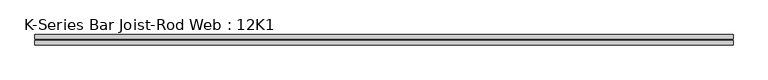
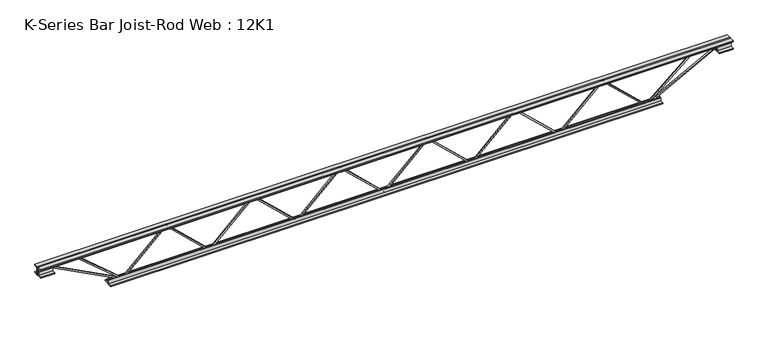
"""IFC4 building model written with IfcOpenShell, lengths in millimetres: beam geometry, K-Series Bar Joist-Rod Web : 12K1."""

from ifc_helpers import new_model, si_unit, frame, origin, place, context, project, spatial, polyline, outline, extrude, source, transform, mapped, element, save


def k_series_bar_joist_rod_web_12k1_562b93e1(model_context):
    return source(origin(), model_context, "Body", "SweptSolid", [
        extrude(outline(polyline([(-141.2875, 631.2958333), (-150.8125, 631.2958333), (-150.8125, 636.3642323), (141.2875, 945.662149), (141.2875, 948.225351), (-150.8125, 1257.5232677), (-150.8125, 1262.5916667), (-141.2875, 1262.5916667), (-141.2875, 1261.3100656), (150.8125, 952.012149), (150.8125, 941.875351), (-141.2875, 632.5774344), (-141.2875, 631.2958333)])), frame((0.0, -4.7625, 0.0), z_axis=(0.0, 1.0, 0.0), x_axis=(0.0, 0.0, 1.0)), (0.0, 0.0, 1.0), 9.525),
        extrude(outline(polyline([(-141.2875, 0.0), (-150.8125, 0.0), (-150.8125, 5.068399), (141.2875, 314.3663156), (141.2875, 316.9295177), (-150.8125, 626.2274344), (-150.8125, 631.2958333), (-141.2875, 631.2958333), (-141.2875, 630.0142323), (150.8125, 320.7163156), (150.8125, 310.5795177), (-141.2875, 1.281601), (-141.2875, 0.0)])), frame((0.0, -4.7625, 0.0), z_axis=(0.0, 1.0, 0.0), x_axis=(0.0, 0.0, 1.0)), (0.0, 0.0, 1.0), 9.525),
        extrude(outline(polyline([(-141.2875, -631.2958333), (-150.8125, -631.2958333), (-150.8125, -626.2274344), (141.2875, -316.9295177), (141.2875, -314.3663156), (-150.8125, -5.068399), (-150.8125, 0.0), (-141.2875, 0.0), (-141.2875, -1.281601), (150.8125, -310.5795177), (150.8125, -320.7163156), (-141.2875, -630.0142323), (-141.2875, -631.2958333)])), frame((0.0, -4.7625, 0.0), z_axis=(0.0, 1.0, 0.0), x_axis=(0.0, 0.0, 1.0)), (0.0, 0.0, 1.0), 9.525),
        extrude(outline(polyline([(-141.2875, -1262.5916667), (-150.8125, -1262.5916667), (-150.8125, -1257.5232677), (141.2875, -948.225351), (141.2875, -945.662149), (-150.8125, -636.3642323), (-150.8125, -631.2958333), (-141.2875, -631.2958333), (-141.2875, -632.5774344), (150.8125, -941.875351), (150.8125, -952.012149), (-141.2875, -1261.3100656), (-141.2875, -1262.5916667)])), frame((0.0, -4.7625, 0.0), z_axis=(0.0, 1.0, 0.0), x_axis=(0.0, 0.0, 1.0)), (0.0, 0.0, 1.0), 9.525),
        extrude(outline(polyline([(-141.2875, 1262.5916667), (-150.8125, 1262.5916667), (-150.8125, 1267.6600656), (141.2875, 1576.9579823), (141.2875, 1579.5211844), (-150.8125, 1888.819101), (-150.8125, 1893.8875), (-141.2875, 1893.8875), (-141.2875, 1892.605899), (150.8125, 1583.3079823), (150.8125, 1573.1711844), (-141.2875, 1263.8732677), (-141.2875, 1262.5916667)])), frame((0.0, -4.7625, 0.0), z_axis=(0.0, 1.0, 0.0), x_axis=(0.0, 0.0, 1.0)), (0.0, 0.0, 1.0), 9.525),
        extrude(outline(polyline([(-141.2875, -1893.8875), (-150.8125, -1893.8875), (-150.8125, -1888.819101), (141.2875, -1579.5211844), (141.2875, -1576.9579823), (-150.8125, -1267.6600656), (-150.8125, -1262.5916667), (-141.2875, -1262.5916667), (-141.2875, -1263.8732677), (150.8125, -1573.1711844), (150.8125, -1583.3079823), (-141.2875, -1892.605899), (-141.2875, -1893.8875)])), frame((0.0, -4.7625, 0.0), z_axis=(0.0, 1.0, 0.0), x_axis=(0.0, 0.0, 1.0)), (0.0, 0.0, 1.0), 9.525),
        extrude(outline(polyline([(4.7625, 152.4), (36.5125, 152.4), (36.5125, 146.05), (11.1125, 146.05), (11.1125, 120.65), (4.7625, 120.65), (4.7625, 152.4)])), frame((-2503.4875, 0.0, 0.0), z_axis=(1.0, 0.0, 0.0), x_axis=(0.0, 1.0, 0.0)), (0.0, 0.0, 1.0), 5006.975),
        extrude(outline(polyline([(-4.7625, 152.4), (-4.7625, 120.65), (-11.1125, 120.65), (-11.1125, 146.05), (-36.5125, 146.05), (-36.5125, 152.4), (-4.7625, 152.4)])), frame((-2503.4875, 0.0, 0.0), z_axis=(1.0, 0.0, 0.0), x_axis=(0.0, 1.0, 0.0)), (0.0, 0.0, 1.0), 5006.975),
        extrude(outline(polyline([(-4.7625, 88.9), (-36.5125, 88.9), (-36.5125, 95.25), (-11.1125, 95.25), (-11.1125, 120.65), (-4.7625, 120.65), (-4.7625, 88.9)])), frame((-2503.4875, 0.0, 0.0), z_axis=(1.0, 0.0, 0.0), x_axis=(0.0, 1.0, 0.0)), (0.0, 0.0, 1.0), 101.6),
        extrude(outline(polyline([(36.5125, 88.9), (4.7625, 88.9), (4.7625, 120.65), (11.1125, 120.65), (11.1125, 95.25), (36.5125, 95.25), (36.5125, 88.9)])), frame((-2503.4875, 0.0, 0.0), z_axis=(1.0, 0.0, 0.0), x_axis=(0.0, 1.0, 0.0)), (0.0, 0.0, 1.0), 101.6),
        extrude(outline(polyline([(4.7625, 88.9), (4.7625, 120.65), (11.1125, 120.65), (11.1125, 95.25), (36.5125, 95.25), (36.5125, 88.9), (4.7625, 88.9)])), frame((2401.8875, 0.0, 0.0), z_axis=(1.0, 0.0, 0.0), x_axis=(0.0, 1.0, 0.0)), (0.0, 0.0, 1.0), 101.6),
        extrude(outline(polyline([(-4.7625, 88.9), (-36.5125, 88.9), (-36.5125, 95.25), (-11.1125, 95.25), (-11.1125, 120.65), (-4.7625, 120.65), (-4.7625, 88.9)])), frame((2401.8875, 0.0, 0.0), z_axis=(1.0, 0.0, 0.0), x_axis=(0.0, 1.0, 0.0)), (0.0, 0.0, 1.0), 101.6),
        extrude(outline(polyline([(4.7625, -152.4), (4.7625, -120.65), (11.1125, -120.65), (11.1125, -146.05), (36.5125, -146.05), (36.5125, -152.4), (4.7625, -152.4)])), frame((-1995.4875, 0.0, 0.0), z_axis=(1.0, 0.0, 0.0), x_axis=(0.0, 1.0, 0.0)), (0.0, 0.0, 1.0), 3990.975),
        extrude(outline(polyline([(-4.7625, -152.4), (-36.5125, -152.4), (-36.5125, -146.05), (-11.1125, -146.05), (-11.1125, -120.65), (-4.7625, -120.65), (-4.7625, -152.4)])), frame((-1995.4875, 0.0, 0.0), z_axis=(1.0, 0.0, 0.0), x_axis=(0.0, 1.0, 0.0)), (0.0, 0.0, 1.0), 3990.975),
        extrude(outline(polyline([(0.0, -9.525), (0.0, 0.0), (573.7533355, 0.0), (573.7533355, -9.525), (0.0, -9.525)])), frame((-2404.1012714, 4.7625, 116.4332925), z_axis=(0.4648338989895134, 0.0, 0.8853979028381572), x_axis=(0.8853979028381572, 0.0, -0.4648338989895134)), (0.0, 0.0, 1.0), 9.525),
        extrude(outline(polyline([(0.0, -9.525), (0.0, 0.0), (413.2341918, 0.0), (413.2341918, -9.525), (0.0, -9.525)])), frame((-2212.6091186, 4.7625, 117.0121761), z_axis=(0.6453967393642932, 0.0, 0.7638475298238114), x_axis=(0.7638475298238114, 0.0, -0.6453967393642932)), (0.0, 0.0, 1.0), 9.525),
        extrude(outline(polyline([(0.0, -9.525), (0.0, 0.0), (573.7533355, 0.0), (573.7533355, -9.525), (0.0, -9.525)])), frame((2404.1012714, -4.7625, 116.4332925), z_axis=(-0.46483389898949556, 0.0, 0.8853979028381666), x_axis=(-0.8853979028381666, 0.0, -0.46483389898949556)), (0.0, 0.0, 1.0), 9.525),
        extrude(outline(polyline([(0.0, -9.525), (0.0, 0.0), (413.2341918, 0.0), (413.2341918, -9.525), (0.0, -9.525)])), frame((2212.6091186, -4.7625, 117.0121761), z_axis=(-0.6453967393642873, 0.0, 0.7638475298238165), x_axis=(-0.7638475298238165, 0.0, -0.6453967393642873)), (0.0, 0.0, 1.0), 9.525),
    ])


if __name__ == "__main__":
    model = new_model("IFC4")
    model_context = context("Model", 3, world=origin())
    ifc_project = project(units=[si_unit("LENGTHUNIT", "METRE", prefix="MILLI")], contexts=[model_context])
    site = spatial("IfcSite", under=ifc_project)
    building = spatial("IfcBuilding", under=site)
    placement = place(None, origin())
    k_series_bar_joist_rod_web_12k1_shape = k_series_bar_joist_rod_web_12k1_562b93e1(model_context)
    element("IfcBeam", 1, ObjectType="K-Series Bar Joist-Rod Web : 12K1", at=placement, inside=building, context=model_context, shape_type="MappedRepresentation", body=[
        mapped(k_series_bar_joist_rod_web_12k1_shape, transform((0.0, 0.0, 0.0), x_axis=(1.0, 0.0, 0.0), y_axis=(0.0, 1.0, 0.0), z_axis=(0.0, 0.0, 1.0))),
    ])
    save(model, "model.ifc")

# Revit data of these elements
# Type "K-Series Bar Joist-Rod Web : 12K1"
#   Assembly Code = "B1010350"
#   Wt = 5
#   Web Thickness = 9.525 mm
#   Start Offset [instance default] = 0 mm
#   Start Extension [instance default] = 0 mm
#   Seat Length = 101.6 mm
#   Seat Depth = 63.5 mm
#   PanelArrayLength [instance default] = 6096 mm
#   Panel [instance default] = 609.6 mm
#   End Offset [instance default] = 0 mm
#   End Extension [instance default] = 0 mm
#   End Panel = 609.6 mm
#   Cord Leg = 31.75 mm
#   Chord Thickness = 6.35 mm
#   Length [instance default] = 7315.2 mm
#   Depth = 304.8 mm
#   PanelArrayNum [instance default] = 10
#   Structural Material = Steel ASTM A500, Grade C, Round
# Element 1 (IfcBeam, "K-Series Bar Joist-Rod Web : 12K1")
#   PanelArrayLength = 3787.775 mm
#   Panel = 631.296 mm
#   PanelArrayNum = 6
#   Materials on its faces: "Steel ASTM A500, Grade C, Round"
# Materials
#   "Steel ASTM A500, Grade C, Round": class "Metal", colour RGB 202 101 0, transparency 0, Description = "Carbon steel", Cost = 0
